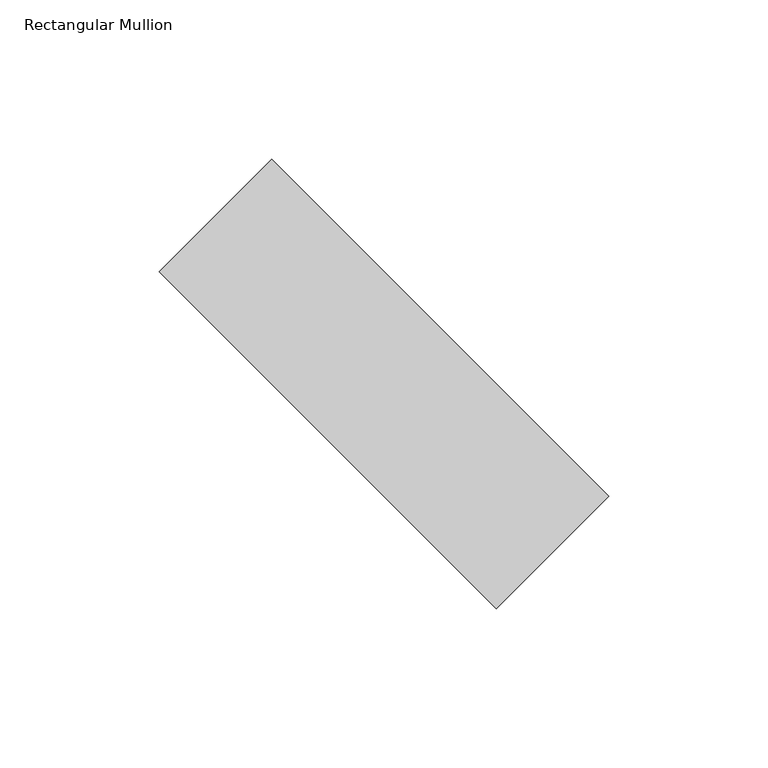
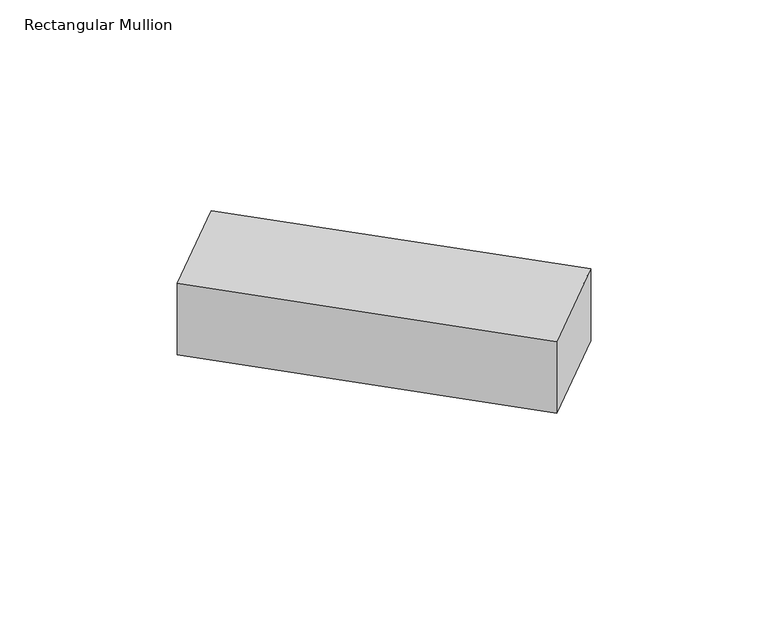
"""IFC4 building model written with IfcOpenShell, lengths in millimetres: member geometry, Rectangular Mullion : tilted mullions."""

from ifc_helpers import new_model, si_unit, frame, origin, place, context, project, spatial, polyline, outline, extrude, source, transform, mapped, element, save


def rectangular_mullion_5612cd03(model_context):
    return source(origin(), model_context, "Body", "SweptSolid", [
        extrude(outline(polyline([(-35.3553391, 70.7106781), (70.7106781, -35.3553391), (35.3553391, -70.7106781), (-70.7106781, 35.3553391), (-35.3553391, 70.7106781)])), frame((0.0, 0.0, -33.406833), z_axis=(0.0, 0.0, 1.0), x_axis=(1.0, 0.0, 0.0)), (0.0, 0.0, 1.0), 33.406833),
    ])


if __name__ == "__main__":
    model = new_model("IFC4")
    model_context = context("Model", 3, world=origin())
    ifc_project = project(units=[si_unit("LENGTHUNIT", "METRE", prefix="MILLI")], contexts=[model_context])
    site = spatial("IfcSite", under=ifc_project)
    building = spatial("IfcBuilding", under=site)
    placement = place(None, origin())
    rectangular_mullion_shape = rectangular_mullion_5612cd03(model_context)
    element("IfcMember", 1, ObjectType="Rectangular Mullion : tilted mullions", at=placement, inside=building, context=model_context, shape_type="MappedRepresentation", body=[
        mapped(rectangular_mullion_shape, transform((0.0, 0.0, 0.0), x_axis=(1.0, 0.0, 0.0), y_axis=(0.0, 1.0, 0.0), z_axis=(0.0, 0.0, 1.0))),
    ])
    save(model, "model.ifc")

# Revit data of these elements
# Type "Rectangular Mullion : tilted mullions"
#   built-in parameter 1007304 = 0.492126 (stored number, unit not read)
#   built-in parameter 1007301 = 0.082021 (stored number, unit not read)
#   built-in parameter 1007300 = 0.082021 (stored number, unit not read)
# Element 1 (IfcMember, "Rectangular Mullion : tilted mullions")
#   Materials on its faces: "Aluminum"
# Materials
#   "Aluminum": class "Metal", colour RGB 244 244 244, transparency 0, Description = "Aluminum 6061", Cost = 0
